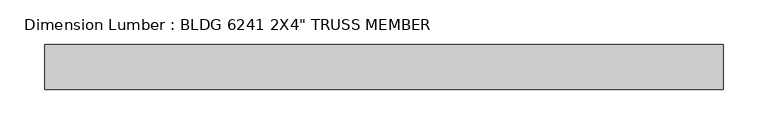
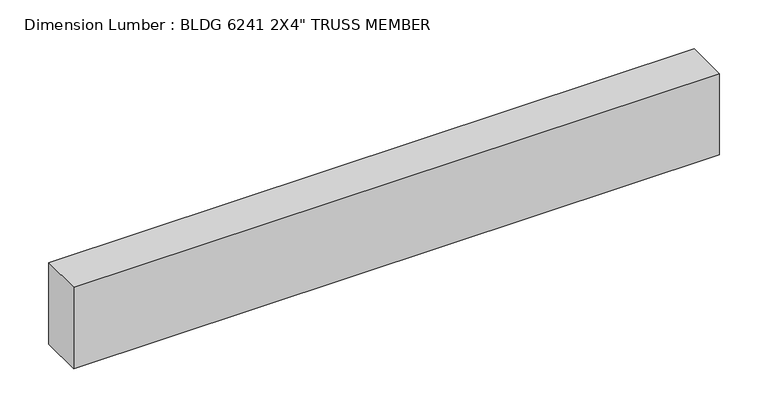
"""IFC4 building model written with IfcOpenShell, lengths in millimetres: beam geometry."""

from ifc_helpers import new_model, si_unit, frame, origin, place, context, project, spatial, polyline, outline, extrude, source, transform, mapped, element, save


def beam_c3ddfe20(model_context):
    return source(origin(), model_context, "Body", "SweptSolid", [
        extrude(outline(polyline([(393.7, 25.4), (393.7, -25.4), (-368.3, -25.4), (-368.3, 25.4), (393.7, 25.4)])), frame((0.0, 0.0, -50.8), z_axis=(0.0, 0.0, 1.0), x_axis=(1.0, 0.0, 0.0)), (0.0, 0.0, 1.0), 101.6),
    ])


if __name__ == "__main__":
    model = new_model("IFC4")
    model_context = context("Model", 3, world=origin())
    ifc_project = project(units=[si_unit("LENGTHUNIT", "METRE", prefix="MILLI")], contexts=[model_context])
    site = spatial("IfcSite", under=ifc_project)
    building = spatial("IfcBuilding", under=site)
    placement = place(None, origin())
    beam_shape = beam_c3ddfe20(model_context)
    element("IfcBeam", 1, ObjectType="Dimension Lumber : BLDG 6241 2X4\" TRUSS MEMBER", at=placement, inside=building, context=model_context, shape_type="MappedRepresentation", body=[
        mapped(beam_shape, transform((0.0, 0.0, 0.0), x_axis=(1.0, 0.0, 0.0), y_axis=(0.0, 1.0, 0.0), z_axis=(0.0, 0.0, 1.0))),
    ])
    save(model, "model.ifc")

# Revit data of these elements
# Type "Dimension Lumber : BLDG 6241 2X4\" TRUSS MEMBER"
#   Assembly Code = "B10"
#   A = 0.273472 SF
#   Length [instance default] = 5' - 0"
#   b = 0' - 2"
#   d = 0' - 4"
#   Structural Material [instance default] = Softwood, Lumber
# Element 1 (IfcBeam, "Dimension Lumber : BLDG 6241 2X4\" TRUSS MEMBER")
#   Materials on its faces: "Softwood, Lumber"
# Materials
#   "Softwood, Lumber": class "Wood", colour RGB 223 192 134, transparency 0, Description = "Pinus Echinata", Cost = 0
